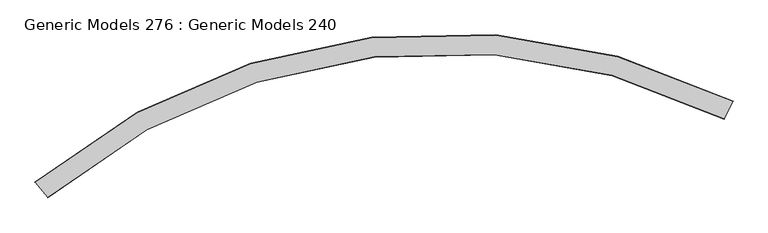
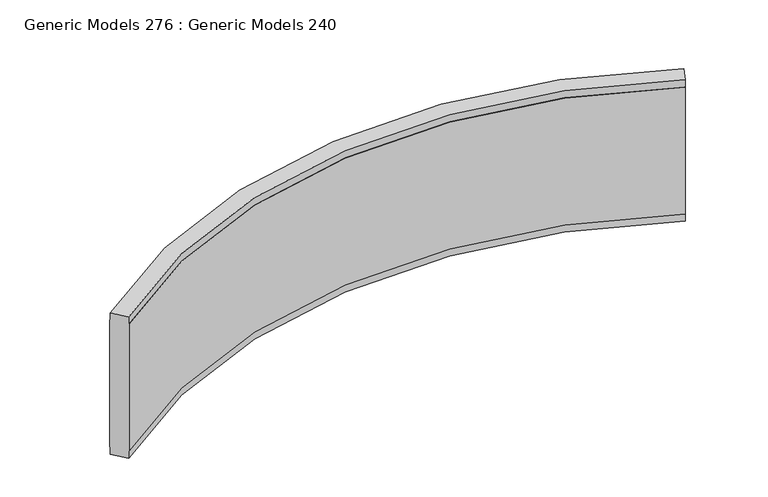
"""IFC4 building model written with IfcOpenShell, lengths in millimetres: proxy geometry, Generic Models 276 : Generic Models 240."""

from ifc_helpers import new_model, si_unit, frame, origin, place, context, project, spatial, polyline, circle_curve, source, transform, mapped, element, save
from ifc_brep_helpers import plane_surface, cylinder_surface, revolved_surface, advanced_brep


def generic_models_276_generic_models_240_3d232618(model_context):
    return source(origin(), model_context, "Body", "AdvancedBrep", [
        advanced_brep(
        [(444.5231527, -22598.0737413, 41.275), (444.5231527, -22598.0737413, 1.5875), (484.4296516, -22518.6339443, 1.5875), (484.4296516, -22518.6339443, 41.275), (485.1457047, -22517.2085346, 41.275), (485.1457047, -22517.2085346, 739.775), (484.4330886, -22518.6271024, 739.775), (484.4330886, -22518.6271024, 779.4625), (444.5265897, -22598.0668994, 779.4625), (444.5265897, -22598.0668994, 739.775), (443.8139737, -22599.4854672, 739.775), (443.8139737, -22599.4854672, 41.275), (-2657.3218922, -22958.51688, 41.275), (-2656.3078884, -22959.7283673, 41.275), (-2656.3078884, -22959.7283673, 739.775), (-2657.3268065, -22958.5110086, 739.775), (-2657.3268065, -22958.5110086, 779.4625), (-2714.3862222, -22890.3389242, 779.4625), (-2714.3862222, -22890.3389242, 739.775), (-2715.4051403, -22889.1215656, 739.775), (-2715.4051403, -22889.1215656, 41.275), (-2714.3813078, -22890.3447957, 41.275), (-2714.3813078, -22890.3447957, 1.5875), (-2657.3218922, -22958.51688, 1.5875)],
        [
            (0, 1),
            (1, 2),
            (2, 3),
            (3, 4),
            (4, 5),
            (5, 6),
            (6, 7),
            (7, 8),
            (8, 9),
            (9, 10),
            (10, 11),
            (11, 0),
            (12, 13),
            (13, 14),
            (14, 15),
            (15, 16),
            (16, 17),
            (17, 18),
            (18, 19),
            (19, 20),
            (20, 21),
            (21, 22),
            (22, 23),
            (23, 12),
            (23, 1, circle_curve(frame((-832.04683, -25139.2753781, 1.5875), z_axis=(0.0, 0.0, -1.0), x_axis=(0.44889200092737946, 0.8935860179654858, 0.0)), 2843.8243053)),
            (0, 12, circle_curve(frame((-832.04683, -25139.2753781, 41.275), z_axis=(0.0, 0.0, 1.0), x_axis=(0.44889200092737946, 0.8935860179654858, 0.0)), 2843.8243053)),
            (22, 2, circle_curve(frame((-832.04683, -25139.2753781, 1.5875), z_axis=(0.0, 0.0, -1.0), x_axis=(0.44889200092737946, 0.8935860179654858, 0.0)), 2932.7243053)),
            (21, 3, circle_curve(frame((-832.04683, -25139.2753781, 41.275), z_axis=(0.0, 0.0, -1.0), x_axis=(0.44889200092737946, 0.8935860179654858, 0.0)), 2932.7243053)),
            (20, 4, circle_curve(frame((-832.04683, -25139.2753781, 41.275), z_axis=(0.0, 0.0, -1.0), x_axis=(0.44889200092737946, 0.8935860179654858, 0.0)), 2934.319462)),
            (19, 5, circle_curve(frame((-832.04683, -25139.2753781, 739.775), z_axis=(0.0, 0.0, -1.0), x_axis=(0.44889200092737946, 0.8935860179654858, 0.0)), 2934.319462)),
            (18, 6, circle_curve(frame((-832.04683, -25139.2753781, 739.775), z_axis=(0.0, 0.0, -1.0), x_axis=(0.44889200092737946, 0.8935860179654858, 0.0)), 2932.731962)),
            (17, 7, circle_curve(frame((-832.04683, -25139.2753781, 779.4625), z_axis=(0.0, 0.0, -1.0), x_axis=(0.44889200092737946, 0.8935860179654858, 0.0)), 2932.731962)),
            (16, 8, circle_curve(frame((-832.04683, -25139.2753781, 779.4625), z_axis=(0.0, 0.0, -1.0), x_axis=(0.44889200092737946, 0.8935860179654858, 0.0)), 2843.831962)),
            (15, 9, circle_curve(frame((-832.04683, -25139.2753781, 739.775), z_axis=(0.0, 0.0, -1.0), x_axis=(0.44889200092737946, 0.8935860179654858, 0.0)), 2843.831962)),
            (14, 10, circle_curve(frame((-832.04683, -25139.2753781, 739.775), z_axis=(0.0, 0.0, -1.0), x_axis=(0.44889200092737946, 0.8935860179654858, 0.0)), 2842.244462)),
            (13, 11, circle_curve(frame((-832.04683, -25139.2753781, 41.275), z_axis=(0.0, 0.0, -1.0), x_axis=(0.44889200092737946, 0.8935860179654858, 0.0)), 2842.244462)),
        ],
        [
            plane_surface(frame((536.1759889, -22415.6251953, -34.925), z_axis=(0.8935860179654859, -0.4488920009273796, 0.0), x_axis=(0.0, 0.0, -1.0))),
            plane_surface(frame((-2788.3696518, -22801.9467711, -34.925), z_axis=(-0.7668400941499618, -0.6418381961242863, 0.0), x_axis=(0.0, 0.0, -1.0))),
            revolved_surface(polyline([(444.523152692032, -22598.07374133351, 41.27499999999999), (444.523152692032, -22598.07374133351, 1.5874999999999986)]), (-832.04683, -25139.2753781, -34.925), (0.0, 0.0, 1.0)),
            plane_surface(frame((-832.04683, -25139.2753781, 1.5875), z_axis=(0.0, 0.0, -1.0000000000000002), x_axis=(0.4488920009273795, 0.8935860179654859, 0.0))),
            cylinder_surface(frame((-832.04683, -25139.2753781, -34.925), z_axis=(0.0, 0.0, 1.0), x_axis=(0.44889200092737946, 0.8935860179654858, 0.0)), 2932.7243053),
            plane_surface(frame((-832.04683, -25139.2753781, 41.275), z_axis=(0.0, 0.0, -1.0000000000000002), x_axis=(0.4488920009273795, 0.8935860179654859, 0.0))),
            cylinder_surface(frame((-832.04683, -25139.2753781, -34.925), z_axis=(0.0, 0.0, 1.0), x_axis=(0.44889200092737946, 0.8935860179654858, 0.0)), 2934.319462),
            plane_surface(frame((-832.04683, -25139.2753781, 739.775), z_axis=(0.0, 0.0, 1.0000000000000002), x_axis=(0.4488920009273795, 0.8935860179654859, 0.0))),
            cylinder_surface(frame((-832.04683, -25139.2753781, -34.925), z_axis=(0.0, 0.0, 1.0), x_axis=(0.44889200092737946, 0.8935860179654858, 0.0)), 2932.731962),
            plane_surface(frame((-832.04683, -25139.2753781, 779.4625), z_axis=(0.0, 0.0, 1.0000000000000002), x_axis=(0.4488920009273795, 0.8935860179654859, 0.0))),
            revolved_surface(polyline([(444.52658972341555, -22598.066899413443, 779.4625), (444.52658972341555, -22598.066899413443, 739.775)]), (-832.04683, -25139.2753781, -34.925), (0.0, 0.0, 1.0)),
            revolved_surface(polyline([(443.81397367194313, -22599.485467216964, 739.775), (443.81397367194313, -22599.485467216964, 41.27499999999999)]), (-832.04683, -25139.2753781, -34.925), (0.0, 0.0, 1.0)),
        ],
        [
            (0, [[1, 2, 3, 4, 5, 6, 7, 8, 9, 10, 11, 12]]),
            (1, [[13, 14, 15, 16, 17, 18, 19, 20, 21, 22, 23, 24]]),
            (2, [[25, -1, 26, -24]]),
            (3, [[27, -2, -25, -23]]),
            (4, [[28, -3, -27, -22]]),
            (5, [[29, -4, -28, -21]]),
            (6, [[30, -5, -29, -20]]),
            (7, [[31, -6, -30, -19]]),
            (8, [[32, -7, -31, -18]]),
            (9, [[33, -8, -32, -17]]),
            (10, [[34, -9, -33, -16]]),
            (7, [[35, -10, -34, -15]]),
            (11, [[36, -11, -35, -14]]),
            (5, [[-26, -12, -36, -13]]),
        ],
    ),
    ])


if __name__ == "__main__":
    model = new_model("IFC4")
    model_context = context("Model", 3, world=origin())
    ifc_project = project(units=[si_unit("LENGTHUNIT", "METRE", prefix="MILLI")], contexts=[model_context])
    site = spatial("IfcSite", under=ifc_project)
    building = spatial("IfcBuilding", under=site)
    placement = place(None, origin())
    generic_models_276_generic_models_240_shape = generic_models_276_generic_models_240_3d232618(model_context)
    element("IfcBuildingElementProxy", 1, Name="Generic Models 276 : Generic Models 240", ObjectType="Generic Models 276 : Generic Models 240", at=placement, inside=building, context=model_context, shape_type="MappedRepresentation", body=[
        mapped(generic_models_276_generic_models_240_shape, transform((0.0, 0.0, 0.0), x_axis=(1.0, 0.0, 0.0), y_axis=(0.0, 1.0, 0.0), z_axis=(0.0, 0.0, 1.0))),
    ])
    save(model, "model.ifc")

# Revit data of these elements
# Element 1 (IfcBuildingElementProxy, "Generic Models 276 : Generic Models 240")
#   Materials on its faces: "METAL STUDS (MATCH DESK HEIGHT"
# Materials
#   "METAL STUDS (MATCH DESK HEIGHT": class "Unassigned", colour RGB 210 209 208, transparency 0, Keynote = "M05121300.02", Cost = 0
